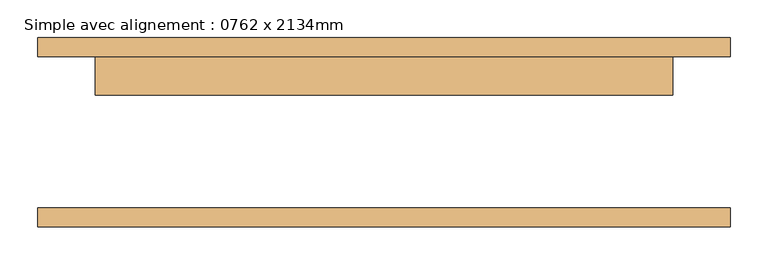
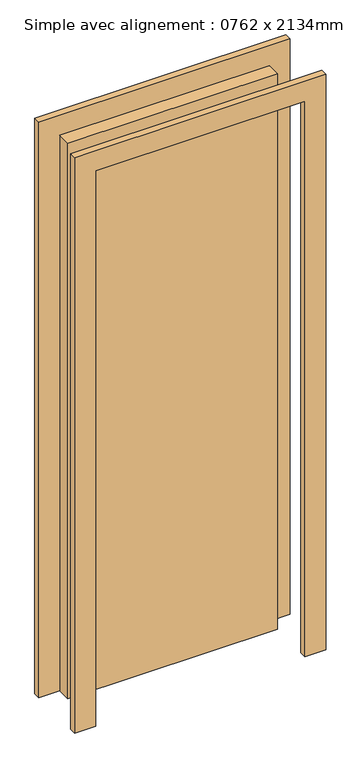
"""IFC4 building model written with IfcOpenShell, lengths in millimetres: door geometry, Simple avec alignement : 0762 x 2134mm."""

from ifc_helpers import new_model, si_unit, frame, origin, origin_with_axes, place, context, project, spatial, polyline, outline, extrude, source, transform, mapped, element, save


def simple_avec_alignement_0762_x_2134mm_85379237(model_context):
    return source(origin(), model_context, "Body", "SweptSolid", [
        extrude(outline(polyline([(2210.0, -457.0), (0.0, -457.0), (0.0, -381.0), (2134.0, -381.0), (2134.0, 381.0), (0.0, 381.0), (0.0, 457.0), (2210.0, 457.0), (2210.0, -457.0)])), frame((0.0, 100.0, 0.0), z_axis=(0.0, 1.0, 0.0), x_axis=(0.0, 0.0, 1.0)), (0.0, 0.0, 1.0), 25.0),
        extrude(outline(polyline([(2210.0, 457.0), (2210.0, -457.0), (0.0, -457.0), (0.0, -381.0), (2134.0, -381.0), (2134.0, 381.0), (0.0, 381.0), (0.0, 457.0), (2210.0, 457.0)])), frame((0.0, -125.0, 0.0), z_axis=(0.0, 1.0, 0.0), x_axis=(0.0, 0.0, 1.0)), (0.0, 0.0, 1.0), 25.0),
        extrude(outline(polyline([(381.0, 49.0), (-381.0, 49.0), (-381.0, 100.0), (381.0, 100.0), (381.0, 49.0)])), origin_with_axes(), (0.0, 0.0, 1.0), 2134.0),
    ])


if __name__ == "__main__":
    model = new_model("IFC4")
    model_context = context("Model", 3, world=origin())
    ifc_project = project(units=[si_unit("LENGTHUNIT", "METRE", prefix="MILLI")], contexts=[model_context])
    site = spatial("IfcSite", under=ifc_project)
    building = spatial("IfcBuilding", under=site)
    placement = place(None, origin())
    simple_avec_alignement_0762_x_2134mm_shape = simple_avec_alignement_0762_x_2134mm_85379237(model_context)
    element("IfcDoor", 1, ObjectType="Simple avec alignement : 0762 x 2134mm", at=placement, inside=building, context=model_context, shape_type="MappedRepresentation", body=[
        mapped(simple_avec_alignement_0762_x_2134mm_shape, transform((0.0, 0.0, 0.0), x_axis=(1.0, 0.0, 0.0), y_axis=(0.0, 1.0, 0.0), z_axis=(0.0, 0.0, 1.0))),
    ])
    save(model, "model.ifc")

# Revit data of these elements
# Type "Simple avec alignement : 0762 x 2134mm"
#   Type Mark = "16"
#   Construction Type Id = "MDOOR"
#   Analytic Construction = "Métal"
#   Thickness = 0.051 m
#   Heat Transfer Coefficient (U) = 3.7021 W/(m²·K)
#   Height = 2.134 m
#   Ajuster la projection Ext = 0.025 m
#   Ajuster la projection Int = 0.025 m
#   Ajuster la largeur = 0.076 m
#   Width = 0.762 m
#   Function = 0
#   Define Thermal Properties by = 1
#   Matériau de porte = Porte - Panneau
#   Matériau des huisseries = Porte - Cadre
#   Visual Light Transmittance = 0
#   Solar Heat Gain Coefficient = 0
#   Function = (empty or 0)
#   Wall Closure = (empty or 0)
# Element 1 (IfcDoor, "Simple avec alignement : 0762 x 2134mm")
#   Materials on its faces: "Porte - Cadre", "Porte - Panneau"
# Materials
#   "Porte - Panneau": class "Bois", colour RGB 210 159 95, transparency 0, Cost = 0
#   "Porte - Cadre": class "Peinture", colour RGB 118 70 51, transparency 0, Cost = 0
